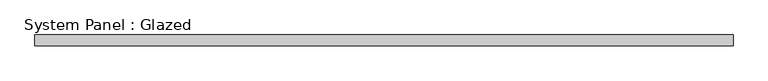
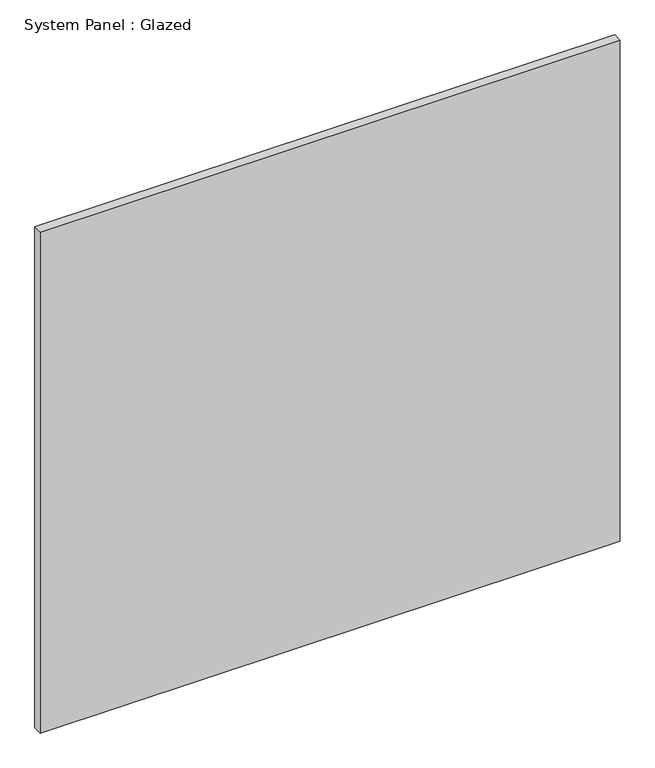
"""IFC4 building model written with IfcOpenShell, lengths in millimetres: plate geometry, System Panel : Glazed."""

from ifc_helpers import new_model, si_unit, origin, origin_with_axes, place, context, project, spatial, polyline, outline, extrude, source, transform, mapped, element, save


def system_panel_glazed_73a2ea9a(model_context):
    return source(origin(), model_context, "Body", "SweptSolid", [
        extrude(outline(polyline([(807.8178526, 24.5), (-807.8178526, 24.5), (-807.8178526, 49.5), (807.8178526, 49.5), (807.8178526, 24.5)])), origin_with_axes(), (0.0, 0.0, 1.0), 1476.6044889),
    ])


if __name__ == "__main__":
    model = new_model("IFC4")
    model_context = context("Model", 3, world=origin())
    ifc_project = project(units=[si_unit("LENGTHUNIT", "METRE", prefix="MILLI")], contexts=[model_context])
    site = spatial("IfcSite", under=ifc_project)
    building = spatial("IfcBuilding", under=site)
    placement = place(None, origin())
    system_panel_glazed_shape = system_panel_glazed_73a2ea9a(model_context)
    element("IfcPlate", 1, ObjectType="System Panel : Glazed", at=placement, inside=building, context=model_context, shape_type="MappedRepresentation", body=[
        mapped(system_panel_glazed_shape, transform((0.0, 0.0, 0.0), x_axis=(1.0, 0.0, 0.0), y_axis=(0.0, 1.0, 0.0), z_axis=(0.0, 0.0, 1.0))),
    ])
    save(model, "model.ifc")

# Revit data of these elements
# Element 1 (IfcPlate, "System Panel : Glazed")
#   Materials on its faces: "Glass"
# Materials
#   "Glass": class "Glass", colour RGB 218 227 224, transparency 0.85, Description = "Soda Lime Glass", Cost = 0
